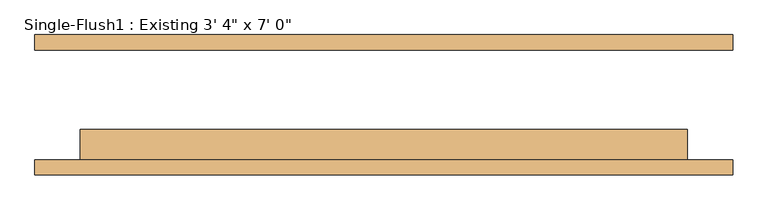
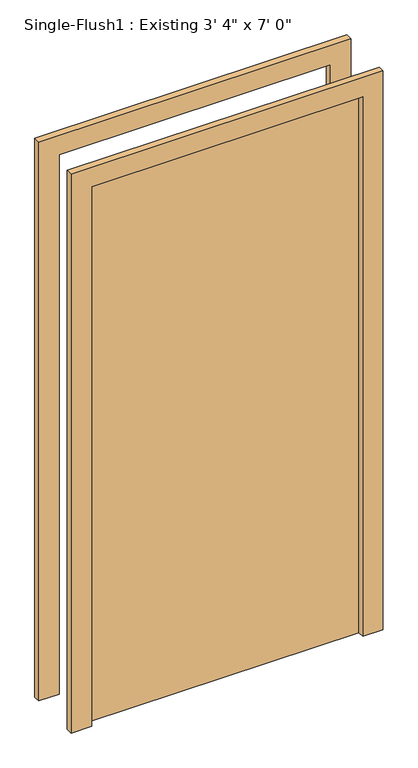
"""IFC4 building model written with IfcOpenShell, lengths in millimetres: door geometry."""

from ifc_helpers import new_model, si_unit, frame, origin, origin_with_axes, place, context, project, spatial, polyline, outline, extrude, source, transform, mapped, element, save


def door_9fd2ff77(model_context):
    return source(origin(), model_context, "Body", "SweptSolid", [
        extrude(outline(polyline([(2209.8, -584.2), (0.0, -584.2), (0.0, -508.0), (2133.6, -508.0), (2133.6, 508.0), (0.0, 508.0), (0.0, 584.2), (2209.8, 584.2), (2209.8, -584.2)])), frame((0.0, -117.475, 0.0), z_axis=(0.0, 1.0, 0.0), x_axis=(0.0, 0.0, 1.0)), (0.0, 0.0, 1.0), 25.4),
        extrude(outline(polyline([(2209.8, 584.2), (2209.8, -584.2), (0.0, -584.2), (0.0, -508.0), (2133.6, -508.0), (2133.6, 508.0), (0.0, 508.0), (0.0, 584.2), (2209.8, 584.2)])), frame((0.0, 92.075, 0.0), z_axis=(0.0, 1.0, 0.0), x_axis=(0.0, 0.0, 1.0)), (0.0, 0.0, 1.0), 25.4),
        extrude(outline(polyline([(508.0, -41.275), (508.0, -92.075), (-508.0, -92.075), (-508.0, -41.275), (508.0, -41.275)])), origin_with_axes(), (0.0, 0.0, 1.0), 2133.6),
    ])


if __name__ == "__main__":
    model = new_model("IFC4")
    model_context = context("Model", 3, world=origin())
    ifc_project = project(units=[si_unit("LENGTHUNIT", "METRE", prefix="MILLI")], contexts=[model_context])
    site = spatial("IfcSite", under=ifc_project)
    building = spatial("IfcBuilding", under=site)
    placement = place(None, origin())
    door_shape = door_9fd2ff77(model_context)
    element("IfcDoor", 1, ObjectType="Single-Flush1 : Existing 3' 4\" x 7' 0\"", at=placement, inside=building, context=model_context, shape_type="MappedRepresentation", body=[
        mapped(door_shape, transform((0.0, 0.0, 0.0), x_axis=(1.0, 0.0, 0.0), y_axis=(0.0, 1.0, 0.0), z_axis=(0.0, 0.0, 1.0))),
    ])
    save(model, "model.ifc")

# Revit data of these elements
# Type "Single-Flush1 : Existing 3' 4\" x 7' 0\""
#   Type Mark = "EX"
#   Construction Type Id = "MDOOR"
#   Assembly Code = "C1020"
#   Analytic Construction = "Metal"
#   Thickness = 0' - 2"
#   Heat Transfer Coefficient (U) = 3.7021 W/(m²·K)
#   Height = 7' - 0"
#   Trim Projection Ext = 0' - 1"
#   Trim Projection Int = 0' - 1"
#   Trim Width = 0' - 3"
#   Width = 3' - 4"
#   Door Material = Door - Panel
#   Frame Material = Door - Frame
#   Visual Light Transmittance = 0
#   Solar Heat Gain Coefficient = 0
#   Function = (empty or 0)
#   Wall Closure = (empty or 0)
# Element 1 (IfcDoor, "Single-Flush1 : Existing 3' 4\" x 7' 0\"")
#   Materials on its faces: "Door - Frame", "Door - Panel"
# Materials
#   "Door - Panel": class "Wood", colour RGB 255 255 255, transparency 0, Cost = 0
#   "Door - Frame": class "Miscellaneous", colour RGB 255 255 255, transparency 0, Cost = 0
